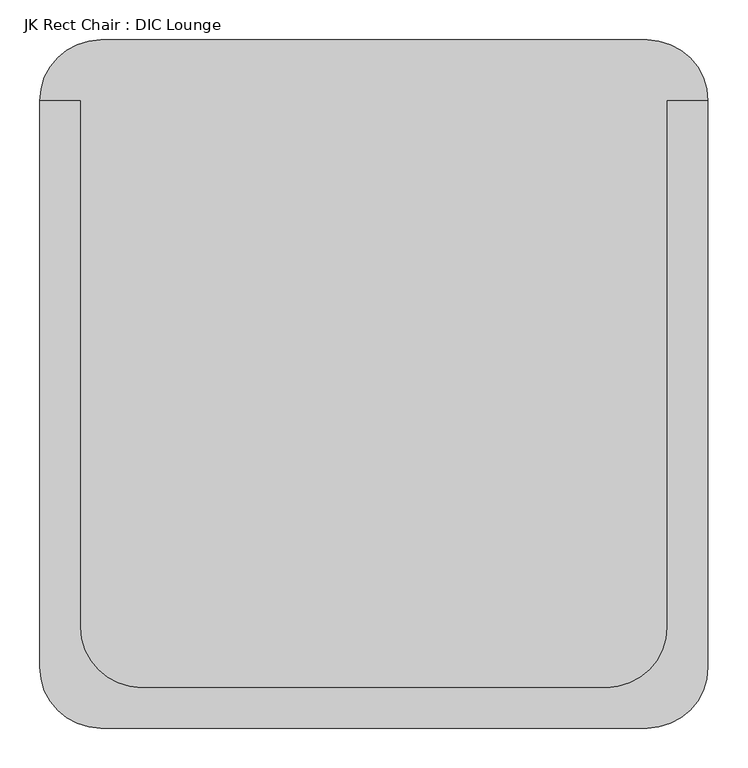
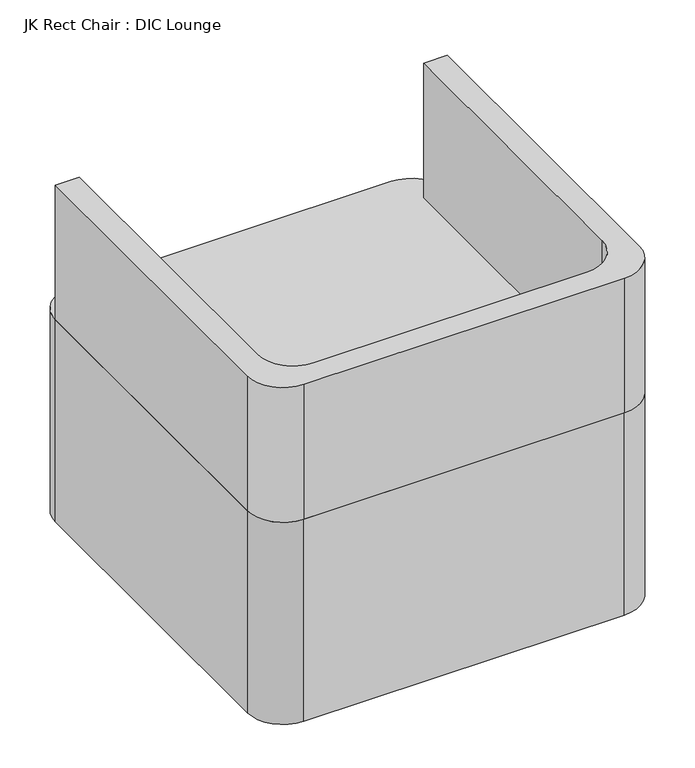
"""IFC4 building model written with IfcOpenShell, lengths in millimetres: furniture geometry, JK Rect Chair : DIC Lounge."""

from ifc_helpers import new_model, si_unit, point, frame, frame_2d, origin, origin_with_axes, place, context, project, spatial, polyline, circle_curve, trimmed, segment, composite_curve, outline, extrude, source, transform, mapped, element, save


def jk_rect_chair_dic_lounge_a5408af2(model_context):
    return source(origin(), model_context, "Body", "SweptSolid", [
        extrude(outline(composite_curve([segment(polyline([(-430.2426335, 322.0544704), (-430.2426335, -338.3455296)]), True, "CONTINUOUS"), segment(trimmed(circle_curve(frame_2d((-354.0426335, -338.3455296)), 76.2), [point((-430.2426335, -338.3455296))], [point((-354.0426335, -414.5455296))], True, "CARTESIAN"), True, "CONTINUOUS"), segment(polyline([(-354.0426335, -414.5455296), (230.1573665, -414.5455296)]), True, "CONTINUOUS"), segment(trimmed(circle_curve(frame_2d((230.1573665, -338.3455296)), 76.2), [point((230.1573665, -414.5455296))], [point((306.3573665, -338.3455296))], True, "CARTESIAN"), True, "CONTINUOUS"), segment(polyline([(306.3573665, -338.3455296), (306.3573665, 322.0544704), (357.1573665, 322.0544704), (357.1573665, -389.1455296)]), True, "CONTINUOUS"), segment(trimmed(circle_curve(frame_2d((280.9573665, -389.1455296)), 76.2), [point((357.1573665, -389.1455296))], [point((280.9573665, -465.3455296))], False, "CARTESIAN"), True, "CONTINUOUS"), segment(polyline([(280.9573665, -465.3455296), (-404.8426335, -465.3455296)]), True, "CONTINUOUS"), segment(trimmed(circle_curve(frame_2d((-404.8426335, -389.1455296)), 76.2), [point((-404.8426335, -465.3455296))], [point((-481.0426335, -389.1455296))], False, "CARTESIAN"), True, "CONTINUOUS"), segment(polyline([(-481.0426335, -389.1455296), (-481.0426335, 322.0544704), (-430.2426335, 322.0544704)]), True, "CONTINUOUS")], self_intersect=False)), frame((0.0, 0.0, 457.2), z_axis=(0.0, 0.0, 1.0), x_axis=(1.0, 0.0, 0.0)), (0.0, 0.0, 1.0), 304.8),
        extrude(outline(composite_curve([segment(polyline([(-481.0426335, -389.1455296), (-481.0426335, 322.0544704)]), True, "CONTINUOUS"), segment(trimmed(circle_curve(frame_2d((-404.8426335, 322.0544704)), 76.2), [point((-481.0426335, 322.0544704))], [point((-404.8426335, 398.2544704))], False, "CARTESIAN"), True, "CONTINUOUS"), segment(polyline([(-404.8426335, 398.2544704), (280.9573665, 398.2544704)]), True, "CONTINUOUS"), segment(trimmed(circle_curve(frame_2d((280.9573665, 322.0544704)), 76.2), [point((280.9573665, 398.2544704))], [point((357.1573665, 322.0544704))], False, "CARTESIAN"), True, "CONTINUOUS"), segment(polyline([(357.1573665, 322.0544704), (357.1573665, -389.1455296)]), True, "CONTINUOUS"), segment(trimmed(circle_curve(frame_2d((280.9573665, -389.1455296)), 76.2), [point((357.1573665, -389.1455296))], [point((280.9573665, -465.3455296))], False, "CARTESIAN"), True, "CONTINUOUS"), segment(polyline([(280.9573665, -465.3455296), (-404.8426335, -465.3455296)]), True, "CONTINUOUS"), segment(trimmed(circle_curve(frame_2d((-404.8426335, -389.1455296)), 76.2), [point((-404.8426335, -465.3455296))], [point((-481.0426335, -389.1455296))], False, "CARTESIAN"), True, "CONTINUOUS")], self_intersect=False)), origin_with_axes(), (0.0, 0.0, 1.0), 457.2),
    ])


if __name__ == "__main__":
    model = new_model("IFC4")
    model_context = context("Model", 3, world=origin())
    ifc_project = project(units=[si_unit("LENGTHUNIT", "METRE", prefix="MILLI")], contexts=[model_context])
    site = spatial("IfcSite", under=ifc_project)
    building = spatial("IfcBuilding", under=site)
    placement = place(None, origin())
    jk_rect_chair_dic_lounge_shape = jk_rect_chair_dic_lounge_a5408af2(model_context)
    element("IfcFurniture", 1, ObjectType="JK Rect Chair : DIC Lounge", at=placement, inside=building, context=model_context, shape_type="MappedRepresentation", body=[
        mapped(jk_rect_chair_dic_lounge_shape, transform((0.0, 0.0, 0.0), x_axis=(1.0, 0.0, 0.0), y_axis=(0.0, 1.0, 0.0), z_axis=(0.0, 0.0, 1.0))),
    ])
    save(model, "model.ifc")

# Revit data of these elements
# Type "JK Rect Chair : DIC Lounge"
#   Width = 2' - 9"
#   Seat Height = 1' - 6"
#   Depth = 2' - 10"
#   Corner Radius = 0' - 3"
#   Back Height = 2' - 6"
#   Status [instance default] = none
#   Default Elevation = 0
